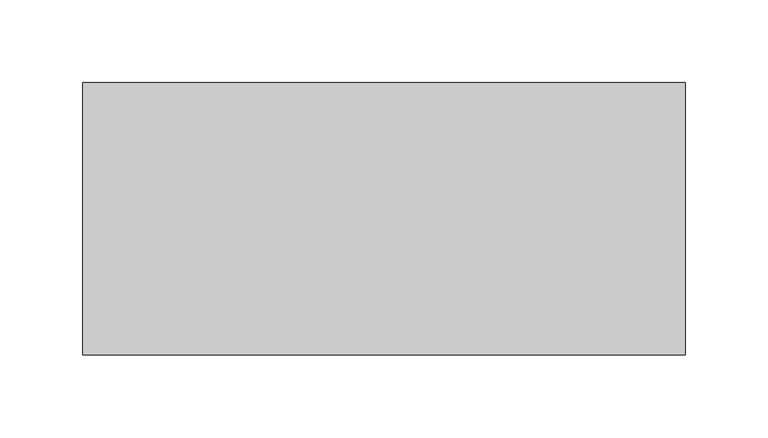
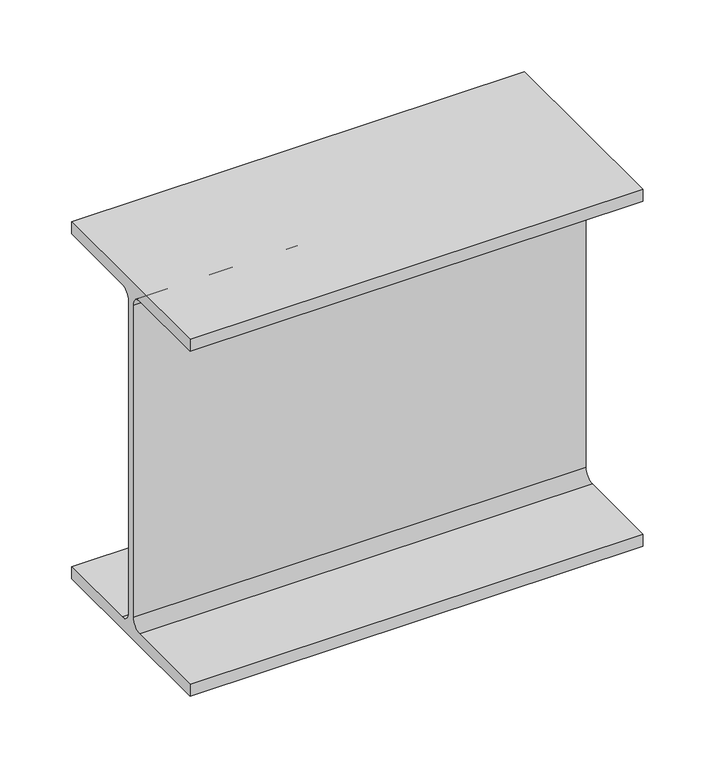
"""IFC4 building model written with IfcOpenShell, lengths in millimetres: beam geometry, Old_Steel Beam_H-KSD3502 : H_SB_ASB_H-300×150x6.5x9."""

from ifc_helpers import new_model, si_unit, point, frame, frame_2d, origin, place, context, project, spatial, polyline, circle_curve, trimmed, segment, composite_curve, outline, extrude, source, transform, mapped, element, save


def beam_8f73eb05(model_context):
    return source(origin(), model_context, "Body", "SweptSolid", [
        extrude(outline(composite_curve([segment(polyline([(82.5, -141.5), (82.5, -151.7), (-82.5, -151.7), (-82.5, -141.5), (-11.9, -141.5)]), True, "CONTINUOUS"), segment(trimmed(circle_curve(frame_2d((-11.9, -132.6)), 8.9), [point((-11.9, -141.5))], [point((-3.0, -132.6))], True, "CARTESIAN"), True, "CONTINUOUS"), segment(polyline([(-3.0, -132.6), (-3.0, 132.6)]), True, "CONTINUOUS"), segment(trimmed(circle_curve(frame_2d((-11.9, 132.6)), 8.9), [point((-3.0, 132.6))], [point((-11.9, 141.5))], True, "CARTESIAN"), True, "CONTINUOUS"), segment(polyline([(-11.9, 141.5), (-82.5, 141.5), (-82.5, 151.7), (82.5, 151.7), (82.5, 141.5), (11.9, 141.5)]), True, "CONTINUOUS"), segment(trimmed(circle_curve(frame_2d((11.9, 132.6)), 8.9), [point((11.9, 141.5))], [point((3.0, 132.6))], True, "CARTESIAN"), True, "CONTINUOUS"), segment(polyline([(3.0, 132.6), (3.0, -132.6)]), True, "CONTINUOUS"), segment(trimmed(circle_curve(frame_2d((11.9, -132.6)), 8.9), [point((3.0, -132.6))], [point((11.9, -141.5))], True, "CARTESIAN"), True, "CONTINUOUS"), segment(polyline([(11.9, -141.5), (82.5, -141.5)]), True, "CONTINUOUS")], self_intersect=False)), frame((-257.2999994, 0.0, 0.0), z_axis=(1.0, 0.0, 0.0), x_axis=(0.0, 1.0, 0.0)), (0.0, 0.0, 1.0), 364.5999994),
    ])


if __name__ == "__main__":
    model = new_model("IFC4")
    model_context = context("Model", 3, world=origin())
    ifc_project = project(units=[si_unit("LENGTHUNIT", "METRE", prefix="MILLI")], contexts=[model_context])
    site = spatial("IfcSite", under=ifc_project)
    building = spatial("IfcBuilding", under=site)
    placement = place(None, origin())
    beam_shape = beam_8f73eb05(model_context)
    element("IfcBeam", 1, ObjectType="Old_Steel Beam_H-KSD3502 : H_SB_ASB_H-300×150x6.5x9", at=placement, inside=building, context=model_context, shape_type="MappedRepresentation", body=[
        mapped(beam_shape, transform((0.0, 0.0, 0.0), x_axis=(1.0, 0.0, 0.0), y_axis=(0.0, 1.0, 0.0), z_axis=(0.0, 0.0, 1.0))),
    ])
    save(model, "model.ifc")

# Revit data of these elements
# Type "Old_Steel Beam_H-KSD3502 : H_SB_ASB_H-300×150x6.5x9"
#   Width = 15.0 cm
#   Web Thickness = 0.65 cm
#   Web Fillet = 1.3 cm
#   Warping Constant = 107174.0 cm⁶
#   Torsional Moment of Inertia = 9.9539 cm⁴
#   Torsional Modulus = 1.0 cm³
#   Section Area = 46.78 cm²
#   Plastic Modulus weak axis = 105.0 cm³
#   Plastic Modulus strong axis = 542.0 cm³
#   Perimeter = 1.17 m²/m
#   Nominal Weight = 36.70 kgf/m
#   Moment of Inertia weak axis = 508.00 cm⁴
#   Moment of Inertia strong axis = 7210.00 cm⁴
#   Height = 30.0 cm
#   Flange Thickness = 0.9 cm
#   Elastic Modulus weak axis = 67.7 cm³
#   Elastic Modulus strong axis = 481.0 cm³
#   Centroid Vertical = 15.0 cm
#   Centroid Horizontal = 7.5 cm
#   Length [instance default] = 1.5240 m
#   Structural Material [instance default] = Steel, 45-345
#   Assembly Code = ""
# Element 1 (IfcBeam, "Old_Steel Beam_H-KSD3502 : H_SB_ASB_H-300×150x6.5x9")
#   Structural Material = none
# Materials
#   "Steel, 45-345": class "Metal", colour RGB 189 187 185, transparency 0, Description = "Steel 345 MPa", Cost = 0
